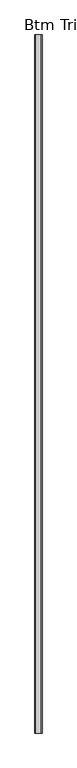
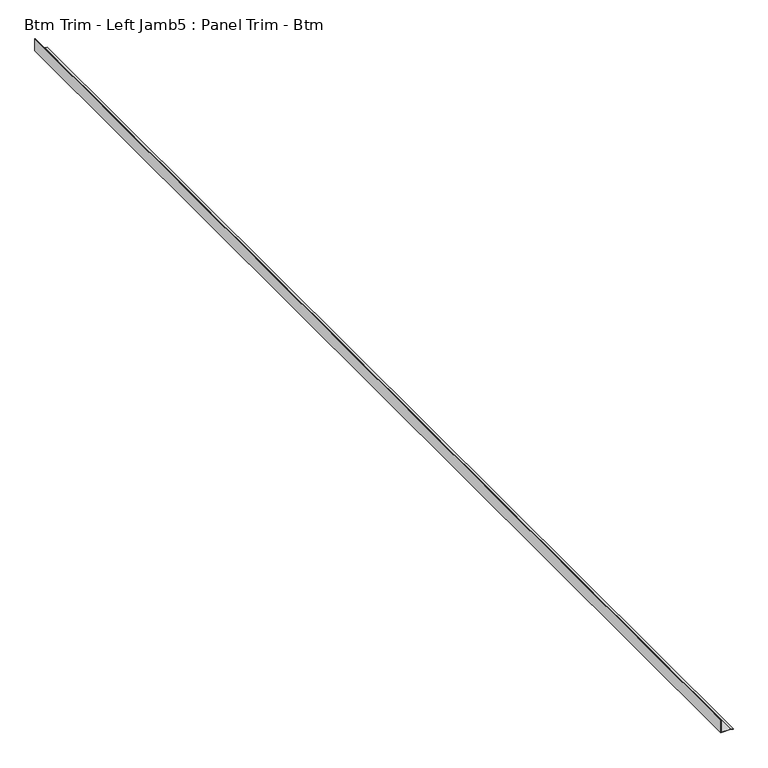
"""IFC4 building model written with IfcOpenShell, lengths in millimetres: proxy geometry, Btm Trim - Left Jamb5 : Panel Trim - Btm."""

from ifc_helpers import new_model, si_unit, frame, origin, place, context, project, spatial, polyline, outline, extrude, source, transform, mapped, element, save


def btm_trim_left_jamb5_panel_trim_btm_415e01f6(model_context):
    return source(origin(), model_context, "Body", "SweptSolid", [
        extrude(outline(polyline([(0.79375, 590391.7729731), (0.79375, 590352.7810739), (51.59375, 590352.7810739), (51.59375, 590351.9936739), (0.0, 590351.9936739), (0.0, 590391.6684739), (-2.4652514, 590400.8689174), (-1.6985478, 590401.074355), (0.79375, 590391.7729731)])), frame((0.0, -536419.2866763, 0.0), z_axis=(0.0, 1.0, 0.0), x_axis=(0.0, 0.0, 1.0)), (0.0, 0.0, 1.0), 4817.5606922),
    ])


if __name__ == "__main__":
    model = new_model("IFC4")
    model_context = context("Model", 3, world=origin())
    ifc_project = project(units=[si_unit("LENGTHUNIT", "METRE", prefix="MILLI")], contexts=[model_context])
    site = spatial("IfcSite", under=ifc_project)
    building = spatial("IfcBuilding", under=site)
    placement = place(None, origin())
    btm_trim_left_jamb5_panel_trim_btm_shape = btm_trim_left_jamb5_panel_trim_btm_415e01f6(model_context)
    element("IfcBuildingElementProxy", 1, Name="Btm Trim - Left Jamb5 : Panel Trim - Btm", ObjectType="Btm Trim - Left Jamb5 : Panel Trim - Btm", at=placement, inside=building, context=model_context, shape_type="MappedRepresentation", body=[
        mapped(btm_trim_left_jamb5_panel_trim_btm_shape, transform((0.0, 0.0, 0.0), x_axis=(1.0, 0.0, 0.0), y_axis=(0.0, 1.0, 0.0), z_axis=(0.0, 0.0, 1.0))),
    ])
    save(model, "model.ifc")

# Revit data of these elements
# Element 1 (IfcBuildingElementProxy, "Btm Trim - Left Jamb5 : Panel Trim - Btm")
#   Materials on its faces: "BASE TRIM BY MTL PANEL MFR."
# Materials
#   "BASE TRIM BY MTL PANEL MFR.": class "Generic", colour RGB 239 242 240, transparency 0, Cost = 0
